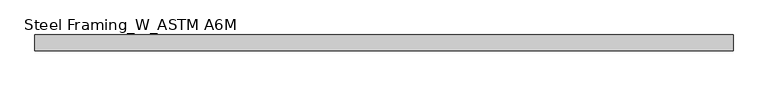
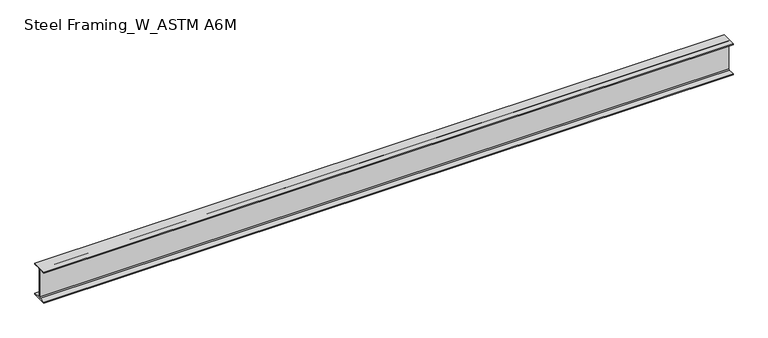
"""IFC4 building model written with IfcOpenShell, lengths in millimetres: beam geometry, Steel Framing_W_ASTM A6M : H_SB_AR_S02_W360x51_G3."""

from ifc_helpers import new_model, si_unit, point, frame, frame_2d, origin, place, context, project, spatial, polyline, circle_curve, trimmed, segment, composite_curve, outline, extrude, source, transform, mapped, element, save


def steel_framing_w_astm_a6m_5f06bcad(model_context):
    return source(origin(), model_context, "Body", "SweptSolid", [
        extrude(outline(composite_curve([segment(polyline([(85.5, -166.4), (85.5, -178.0), (-85.5, -178.0), (-85.5, -166.4), (-13.72, -166.4)]), True, "CONTINUOUS"), segment(trimmed(circle_curve(frame_2d((-13.72, -156.3)), 10.1), [point((-13.72, -166.4))], [point((-3.62, -156.3))], True, "CARTESIAN"), True, "CONTINUOUS"), segment(polyline([(-3.62, -156.3), (-3.62, 156.3)]), True, "CONTINUOUS"), segment(trimmed(circle_curve(frame_2d((-13.72, 156.3)), 10.1), [point((-3.62, 156.3))], [point((-13.72, 166.4))], True, "CARTESIAN"), True, "CONTINUOUS"), segment(polyline([(-13.72, 166.4), (-85.5, 166.4), (-85.5, 178.0), (85.5, 178.0), (85.5, 166.4), (13.72, 166.4)]), True, "CONTINUOUS"), segment(trimmed(circle_curve(frame_2d((13.72, 156.3)), 10.1), [point((13.72, 166.4))], [point((3.62, 156.3))], True, "CARTESIAN"), True, "CONTINUOUS"), segment(polyline([(3.62, 156.3), (3.62, -156.3)]), True, "CONTINUOUS"), segment(trimmed(circle_curve(frame_2d((13.72, -156.3)), 10.1), [point((3.62, -156.3))], [point((13.72, -166.4))], True, "CARTESIAN"), True, "CONTINUOUS"), segment(polyline([(13.72, -166.4), (85.5, -166.4)]), True, "CONTINUOUS")], self_intersect=False)), frame((-3753.8, 0.0, 0.0), z_axis=(1.0, 0.0, 0.0), x_axis=(0.0, 1.0, 0.0)), (0.0, 0.0, 1.0), 7507.6),
    ])


if __name__ == "__main__":
    model = new_model("IFC4")
    model_context = context("Model", 3, world=origin())
    ifc_project = project(units=[si_unit("LENGTHUNIT", "METRE", prefix="MILLI")], contexts=[model_context])
    site = spatial("IfcSite", under=ifc_project)
    building = spatial("IfcBuilding", under=site)
    placement = place(None, origin())
    steel_framing_w_astm_a6m_shape = steel_framing_w_astm_a6m_5f06bcad(model_context)
    element("IfcBeam", 1, ObjectType="Steel Framing_W_ASTM A6M : H_SB_AR_S02_W360x51_G3", at=placement, inside=building, context=model_context, shape_type="MappedRepresentation", body=[
        mapped(steel_framing_w_astm_a6m_shape, transform((0.0, 0.0, 0.0), x_axis=(1.0, 0.0, 0.0), y_axis=(0.0, 1.0, 0.0), z_axis=(0.0, 0.0, 1.0))),
    ])
    save(model, "model.ifc")

# Revit data of these elements
# Type "Steel Framing_W_ASTM A6M : H_SB_AR_S02_W360x51_G3"
#   Type Mark = "G3"
#   Section Name Key = "W14x34"
#   Width = 17.1 cm
#   Web Thickness = 0.724 cm
#   Web Fillet = 1.01 cm
#   Warping Constant = 287000.0 cm⁶
#   Torsional Moment of Inertia = 23.70 cm⁴
#   Section Area = 64.5 cm²
#   Plastic Modulus weak axis = 174.0 cm³
#   Plastic Modulus strong axis = 895.0 cm³
#   Perimeter = 1.36 m²/m
#   Nominal Weight = 51.00 kgf/m
#   Moment of Inertia weak axis = 970.00 cm⁴
#   Moment of Inertia strong axis = 14200.00 cm⁴
#   Height = 35.6 cm
#   Flange Thickness = 1.16 cm
#   Elastic Modulus weak axis = 113.0 cm³
#   Elastic Modulus strong axis = 796.0 cm³
#   Centroid Vertical = 17.8 cm
#   Centroid Horizontal = 8.55 cm
#   Length [instance default] = 1500 mm
#   Structural Material [instance default] = Steel, 45-345
#   Bolt Spacing = 0
#   Assembly Code = ""
# Element 1 (IfcBeam, "Steel Framing_W_ASTM A6M : H_SB_AR_S02_W360x51_G3")
#   Materials on its faces: "Steel, 45-345"
# Materials
#   "Steel, 45-345": class "Metal", colour RGB 189 187 185, transparency 0, Description = "Steel 345 MPa", Cost = 0
